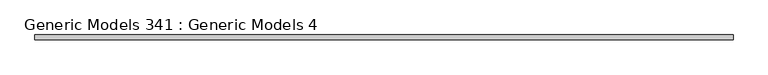
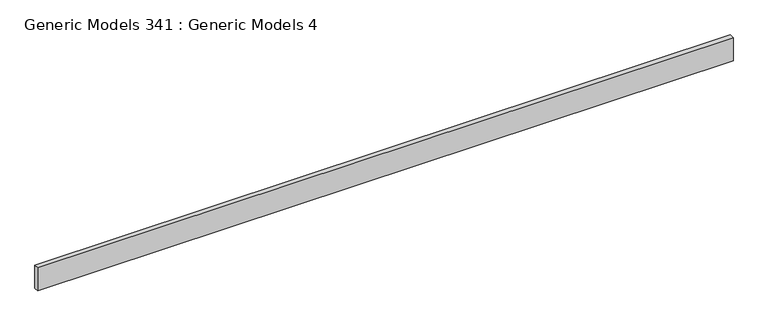
"""IFC4 building model written with IfcOpenShell, lengths in millimetres: proxy geometry, Generic Models 341 : Generic Models 4."""

import ifcopenshell
import ifcopenshell.guid

model = None  # the IFC model being written
_history = None  # IfcOwnerHistory: only IFC2X3 demands one
_inside = {}  # id of a spatial element -> (the spatial element, [elements in it])
_under = {}  # id of a project, library or spatial element -> (it, [spatial elements below it])
_declared = {}  # id of a project -> (the project, [libraries it declares])
_typed = {}  # id of a type object -> (the type object, [elements of that type])
_made_of = {}  # id of a material, layer set ... -> (it, [elements and type objects made of it])


def new_model(schema):
    """Start an empty IFC model of exactly this schema.

    Asked for "IFC4X3", IfcOpenShell would pick the latest addendum, in which some entities
    have other attributes; the version numbers below select the first issue.
    IFC2X3 requires an IfcOwnerHistory on every rooted entity: one is made here for all.
    """
    global model, _history
    if schema == "IFC4X3":
        model = ifcopenshell.file(schema_version=(4, 3, 0, 0))
    else:
        model = ifcopenshell.file(schema=schema)
    _inside.clear()
    _under.clear()
    _declared.clear()
    _typed.clear()
    _made_of.clear()
    _history = None
    if model.schema == "IFC2X3":
        org = make("IfcOrganization", Name="unknown")
        user = make(
            "IfcPersonAndOrganization",
            ThePerson=make("IfcPerson", FamilyName="unknown"),
            TheOrganization=org,
        )
        app = make(
            "IfcApplication",
            ApplicationDeveloper=org,
            Version="unknown",
            ApplicationFullName="unknown",
            ApplicationIdentifier="unknown",
        )
        _history = make(
            "IfcOwnerHistory",
            OwningUser=user,
            OwningApplication=app,
            ChangeAction="ADDED",
            CreationDate=0,
        )
    return model


def make(cls, **values):
    """One entity of the class cls with the attributes given. An attribute that is None is left unset."""
    return model.create_entity(
        cls, **{name: value for name, value in values.items() if value is not None}
    )


def rooted(cls, **values):
    """An entity with a GlobalId (a new one), such as an element, a storey or a relation."""
    return make(cls, GlobalId=ifcopenshell.guid.new(), OwnerHistory=_history, **values)


def si_unit(unit_type, name, prefix=None):
    """IfcSIUnit, for example si_unit("LENGTHUNIT", "METRE", prefix="MILLI")."""
    return make("IfcSIUnit", UnitType=unit_type, Prefix=prefix, Name=name)


def assignment(units):
    """IfcUnitAssignment: the units of a project."""
    return None if units is None else make("IfcUnitAssignment", Units=units)


def point(xyz):
    """IfcCartesianPoint."""
    return None if xyz is None else make("IfcCartesianPoint", Coordinates=xyz)


def direction(xyz):
    """IfcDirection."""
    return None if xyz is None else make("IfcDirection", DirectionRatios=xyz)


def frame(location, z_axis=None, x_axis=None):
    """IfcAxis2Placement3D, a coordinate frame: its origin and axes. An axis left out is left unset."""
    return make(
        "IfcAxis2Placement3D",
        Location=point(location),
        Axis=direction(z_axis),
        RefDirection=direction(x_axis),
    )


def origin():
    """The frame at (0, 0, 0) with its axes left unset."""
    return frame((0.0, 0.0, 0.0))


def place(relative_to, where):
    """IfcLocalPlacement: puts the frame where relative to a parent placement (None: the world)."""
    return make(
        "IfcLocalPlacement", PlacementRelTo=relative_to, RelativePlacement=where
    )


def context(
    kind, dimensions, precision=None, world=None, true_north=None, identifier=None
):
    """IfcGeometricRepresentationContext, for example the 3D "Model" context."""
    return make(
        "IfcGeometricRepresentationContext",
        ContextIdentifier=identifier,
        ContextType=kind,
        CoordinateSpaceDimension=dimensions,
        Precision=precision,
        WorldCoordinateSystem=world,
        TrueNorth=true_north,
    )


def project(units=None, contexts=None):
    """IfcProject with its units and contexts."""
    return rooted(
        "IfcProject",
        Name="project",
        RepresentationContexts=contexts,
        UnitsInContext=assignment(units),
    )


def spatial(cls, under=None, at=None, **own):
    """A site, building, storey or space (cls), placed at a placement, below another one or the project."""
    s = rooted(cls, ObjectPlacement=at, **own)
    if under is not None:
        _under.setdefault(under.id(), (under, []))[1].append(s)
    return s


def polyline(points):
    """IfcPolyline through the points."""
    return make("IfcPolyline", Points=[point(p) for p in points])


def outline(outer, holes=None, kind="AREA"):
    """IfcArbitraryClosedProfileDef: a profile drawn as a closed curve; with holes, ...WithVoids."""
    if holes is None:
        return make("IfcArbitraryClosedProfileDef", ProfileType=kind, OuterCurve=outer)
    return make(
        "IfcArbitraryProfileDefWithVoids",
        ProfileType=kind,
        OuterCurve=outer,
        InnerCurves=holes,
    )


def extrude(swept, where, along, depth):
    """IfcExtrudedAreaSolid: the profile swept, set in the frame where, extruded along a direction by depth."""
    return make(
        "IfcExtrudedAreaSolid",
        SweptArea=swept,
        Position=where,
        ExtrudedDirection=direction(along),
        Depth=depth,
    )


def shape(context_of_items, identifier, shape_type, items):
    """IfcShapeRepresentation: the items that make up one representation, for example the "Body"."""
    return make(
        "IfcShapeRepresentation",
        ContextOfItems=context_of_items,
        RepresentationIdentifier=identifier,
        RepresentationType=shape_type,
        Items=items,
    )


def source(mapping_origin, context_of_items, identifier, shape_type, items):
    """IfcRepresentationMap: a shape defined once, which mapped items show again and again."""
    return make(
        "IfcRepresentationMap",
        MappingOrigin=mapping_origin,
        MappedRepresentation=shape(context_of_items, identifier, shape_type, items),
    )


def transform(
    local_origin,
    x_axis=None,
    y_axis=None,
    z_axis=None,
    scale=None,
    scale2=None,
    scale3=None,
    uniform=True,
):
    """IfcCartesianTransformationOperator3D, or its non-uniform kind. x_axis, y_axis, z_axis: its Axis1, 2, 3."""
    if uniform:
        return make(
            "IfcCartesianTransformationOperator3D",
            Axis1=direction(x_axis),
            Axis2=direction(y_axis),
            LocalOrigin=point(local_origin),
            Scale=scale,
            Axis3=direction(z_axis),
        )
    return make(
        "IfcCartesianTransformationOperator3DnonUniform",
        Axis1=direction(x_axis),
        Axis2=direction(y_axis),
        LocalOrigin=point(local_origin),
        Scale=scale,
        Axis3=direction(z_axis),
        Scale2=scale2,
        Scale3=scale3,
    )


def mapped(mapping_source, mapping_target):
    """IfcMappedItem: shows the shape of a source again, moved by a transform."""
    return make(
        "IfcMappedItem", MappingSource=mapping_source, MappingTarget=mapping_target
    )


def made_of(thing, what):
    """Note that an element or type object is made of a material, layer set ...; save() writes the relation."""
    if what is not None:
        _made_of.setdefault(what.id(), (what, []))[1].append(thing)
    return thing


def element(
    cls,
    number,
    at=None,
    inside=None,
    cuts=None,
    type_object=None,
    material=None,
    context=None,
    identifier="Body",
    shape_type=None,
    held_by="IfcProductDefinitionShape",
    body=None,
    shapes=None,
    **own,
):
    """One element of the class cls, such as IfcWall. Its Tag is "e" and its number.

    at: its placement. inside: the storey or other place that contains it. cuts: it is an
    opening in that element (IfcRelVoidsElement). A single representation is given by context,
    identifier, shape_type and body (its items); several are given by shapes. held_by: the class
    of the entity that holds the representations. save() writes the other relations.
    """
    e = rooted(cls, Tag="e%d" % number, ObjectPlacement=at, **own)
    if body is not None:
        shapes = [shape(context, identifier, shape_type, body)]
    if shapes is not None:
        e.Representation = make(held_by, Representations=shapes)
    if inside is not None:
        _inside.setdefault(inside.id(), (inside, []))[1].append(e)
    if cuts is not None:
        rooted(
            "IfcRelVoidsElement", RelatingBuildingElement=cuts, RelatedOpeningElement=e
        )
    if type_object is not None:
        _typed.setdefault(type_object.id(), (type_object, []))[1].append(e)
    return made_of(e, material)


def aggregate(whole, parts):
    """IfcRelAggregates: a whole, such as a stair, and the parts it consists of."""
    return rooted("IfcRelAggregates", RelatingObject=whole, RelatedObjects=parts)


def save(model, path):
    """Write the relations noted so far, then the file.

    IfcRelAggregates (storeys below a building ...), IfcRelContainedInSpatialStructure (elements
    in a storey), IfcRelDefinesByType, IfcRelAssociatesMaterial and IfcRelDeclares: one each for
    every whole, place, type object, material and project.
    """
    for whole, parts in _under.values():
        aggregate(whole, parts)
    for where, things in _inside.values():
        rooted(
            "IfcRelContainedInSpatialStructure",
            RelatedElements=things,
            RelatingStructure=where,
        )
    for kind, things in _typed.values():
        rooted("IfcRelDefinesByType", RelatedObjects=things, RelatingType=kind)
    for what, things in _made_of.values():
        rooted("IfcRelAssociatesMaterial", RelatedObjects=things, RelatingMaterial=what)
    for by, libraries in _declared.values():
        rooted("IfcRelDeclares", RelatingContext=by, RelatedDefinitions=libraries)
    model.write(path)


def generic_models_341_generic_models_4_3f4d8c2b(model_context):
    return source(origin(), model_context, "Body", "SweptSolid", [
        extrude(outline(polyline([(8383.6828684, 11489.1780759), (8383.6828684, 11361.671352), (-10259.9171316, 11361.671352), (-10259.9171316, 11489.1780759), (8383.6828684, 11489.1780759)])), frame((0.0, 0.0, 126846.6025244), z_axis=(0.0, 0.0, 1.0), x_axis=(1.0, 0.0, 0.0)), (0.0, 0.0, 1.0), 653.3255207),
    ])


if __name__ == "__main__":
    model = new_model("IFC4")
    model_context = context("Model", 3, world=origin())
    ifc_project = project(units=[si_unit("LENGTHUNIT", "METRE", prefix="MILLI")], contexts=[model_context])
    site = spatial("IfcSite", under=ifc_project)
    building = spatial("IfcBuilding", under=site)
    placement = place(None, origin())
    generic_models_341_generic_models_4_shape = generic_models_341_generic_models_4_3f4d8c2b(model_context)
    element("IfcBuildingElementProxy", 1, Name="Generic Models 341 : Generic Models 4", ObjectType="Generic Models 341 : Generic Models 4", at=placement, inside=building, context=model_context, shape_type="MappedRepresentation", body=[
        mapped(generic_models_341_generic_models_4_shape, transform((0.0, 0.0, 0.0), x_axis=(1.0, 0.0, 0.0), y_axis=(0.0, 1.0, 0.0), z_axis=(0.0, 0.0, 1.0))),
    ])
    save(model, "model.ifc")

# Revit data of these elements
# Element 1 (IfcBuildingElementProxy, "Generic Models 341 : Generic Models 4")
#   Materials on its faces: "_BATT INSUL. (U-FACTOR = 0.065 MIN.) OVER CLASS II VAPOR RETARDER(TOWARD INTERIOR)"
# Materials
#   "_BATT INSUL. (U-FACTOR = 0.065 MIN.) OVER CLASS II VAPOR RETARDER(TOWARD INTERIOR)": class "Generic", colour RGB 227 210 251, transparency 0, Cost = 0
